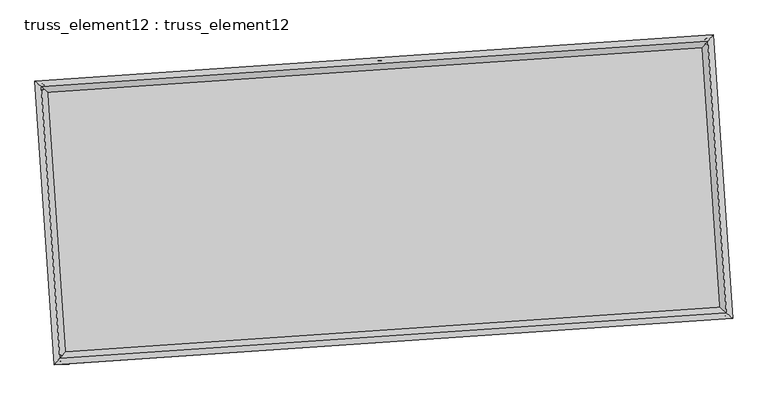
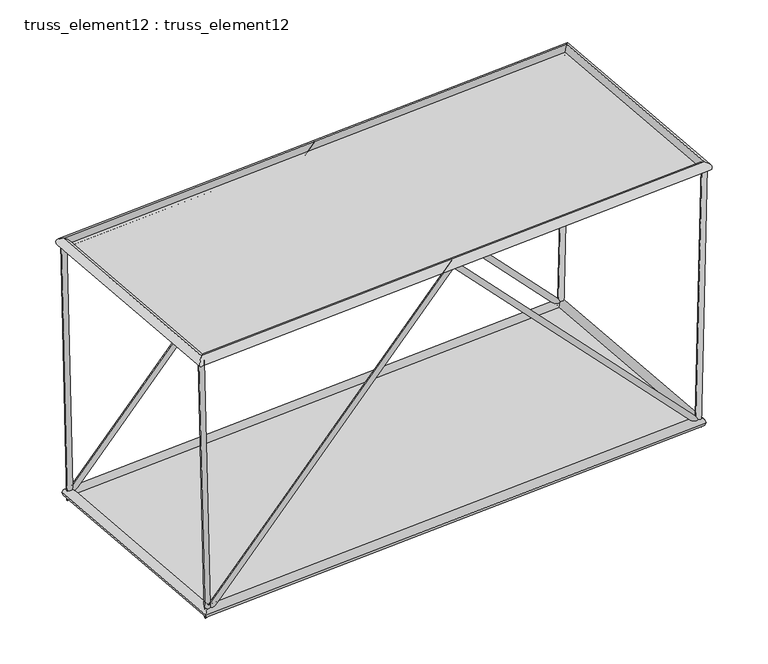
"""IFC4 building model written with IfcOpenShell, lengths in millimetres: plate geometry, truss_element12 : truss_element12."""

import ifcopenshell
import ifcopenshell.guid

model = None  # the IFC model being written
_history = None  # IfcOwnerHistory: only IFC2X3 demands one
_inside = {}  # id of a spatial element -> (the spatial element, [elements in it])
_under = {}  # id of a project, library or spatial element -> (it, [spatial elements below it])
_declared = {}  # id of a project -> (the project, [libraries it declares])
_typed = {}  # id of a type object -> (the type object, [elements of that type])
_made_of = {}  # id of a material, layer set ... -> (it, [elements and type objects made of it])


def new_model(schema):
    """Start an empty IFC model of exactly this schema.

    Asked for "IFC4X3", IfcOpenShell would pick the latest addendum, in which some entities
    have other attributes; the version numbers below select the first issue.
    IFC2X3 requires an IfcOwnerHistory on every rooted entity: one is made here for all.
    """
    global model, _history
    if schema == "IFC4X3":
        model = ifcopenshell.file(schema_version=(4, 3, 0, 0))
    else:
        model = ifcopenshell.file(schema=schema)
    _inside.clear()
    _under.clear()
    _declared.clear()
    _typed.clear()
    _made_of.clear()
    _history = None
    if model.schema == "IFC2X3":
        org = make("IfcOrganization", Name="unknown")
        user = make(
            "IfcPersonAndOrganization",
            ThePerson=make("IfcPerson", FamilyName="unknown"),
            TheOrganization=org,
        )
        app = make(
            "IfcApplication",
            ApplicationDeveloper=org,
            Version="unknown",
            ApplicationFullName="unknown",
            ApplicationIdentifier="unknown",
        )
        _history = make(
            "IfcOwnerHistory",
            OwningUser=user,
            OwningApplication=app,
            ChangeAction="ADDED",
            CreationDate=0,
        )
    return model


def make(cls, **values):
    """One entity of the class cls with the attributes given. An attribute that is None is left unset."""
    return model.create_entity(
        cls, **{name: value for name, value in values.items() if value is not None}
    )


def rooted(cls, **values):
    """An entity with a GlobalId (a new one), such as an element, a storey or a relation."""
    return make(cls, GlobalId=ifcopenshell.guid.new(), OwnerHistory=_history, **values)


def si_unit(unit_type, name, prefix=None):
    """IfcSIUnit, for example si_unit("LENGTHUNIT", "METRE", prefix="MILLI")."""
    return make("IfcSIUnit", UnitType=unit_type, Prefix=prefix, Name=name)


def assignment(units):
    """IfcUnitAssignment: the units of a project."""
    return None if units is None else make("IfcUnitAssignment", Units=units)


def point(xyz):
    """IfcCartesianPoint."""
    return None if xyz is None else make("IfcCartesianPoint", Coordinates=xyz)


def direction(xyz):
    """IfcDirection."""
    return None if xyz is None else make("IfcDirection", DirectionRatios=xyz)


def frame(location, z_axis=None, x_axis=None):
    """IfcAxis2Placement3D, a coordinate frame: its origin and axes. An axis left out is left unset."""
    return make(
        "IfcAxis2Placement3D",
        Location=point(location),
        Axis=direction(z_axis),
        RefDirection=direction(x_axis),
    )


def origin():
    """The frame at (0, 0, 0) with its axes left unset."""
    return frame((0.0, 0.0, 0.0))


def origin_with_axes():
    """The frame at (0, 0, 0) with the z axis (0, 0, 1) and the x axis (1, 0, 0) written out."""
    return frame((0.0, 0.0, 0.0), z_axis=(0.0, 0.0, 1.0), x_axis=(1.0, 0.0, 0.0))


def place(relative_to, where):
    """IfcLocalPlacement: puts the frame where relative to a parent placement (None: the world)."""
    return make(
        "IfcLocalPlacement", PlacementRelTo=relative_to, RelativePlacement=where
    )


def context(
    kind, dimensions, precision=None, world=None, true_north=None, identifier=None
):
    """IfcGeometricRepresentationContext, for example the 3D "Model" context."""
    return make(
        "IfcGeometricRepresentationContext",
        ContextIdentifier=identifier,
        ContextType=kind,
        CoordinateSpaceDimension=dimensions,
        Precision=precision,
        WorldCoordinateSystem=world,
        TrueNorth=true_north,
    )


def project(units=None, contexts=None):
    """IfcProject with its units and contexts."""
    return rooted(
        "IfcProject",
        Name="project",
        RepresentationContexts=contexts,
        UnitsInContext=assignment(units),
    )


def spatial(cls, under=None, at=None, **own):
    """A site, building, storey or space (cls), placed at a placement, below another one or the project."""
    s = rooted(cls, ObjectPlacement=at, **own)
    if under is not None:
        _under.setdefault(under.id(), (under, []))[1].append(s)
    return s


def polyline(points):
    """IfcPolyline through the points."""
    return make("IfcPolyline", Points=[point(p) for p in points])


def circle_curve(where, radius):
    """IfcCircle in the frame where."""
    return make("IfcCircle", Position=where, Radius=radius)


def ellipse_curve(where, semi_axis1, semi_axis2):
    """IfcEllipse in the frame where."""
    return make(
        "IfcEllipse", Position=where, SemiAxis1=semi_axis1, SemiAxis2=semi_axis2
    )


def outline(outer, holes=None, kind="AREA"):
    """IfcArbitraryClosedProfileDef: a profile drawn as a closed curve; with holes, ...WithVoids."""
    if holes is None:
        return make("IfcArbitraryClosedProfileDef", ProfileType=kind, OuterCurve=outer)
    return make(
        "IfcArbitraryProfileDefWithVoids",
        ProfileType=kind,
        OuterCurve=outer,
        InnerCurves=holes,
    )


def extrude(swept, where, along, depth):
    """IfcExtrudedAreaSolid: the profile swept, set in the frame where, extruded along a direction by depth."""
    return make(
        "IfcExtrudedAreaSolid",
        SweptArea=swept,
        Position=where,
        ExtrudedDirection=direction(along),
        Depth=depth,
    )


def shape(context_of_items, identifier, shape_type, items):
    """IfcShapeRepresentation: the items that make up one representation, for example the "Body"."""
    return make(
        "IfcShapeRepresentation",
        ContextOfItems=context_of_items,
        RepresentationIdentifier=identifier,
        RepresentationType=shape_type,
        Items=items,
    )


def source(mapping_origin, context_of_items, identifier, shape_type, items):
    """IfcRepresentationMap: a shape defined once, which mapped items show again and again."""
    return make(
        "IfcRepresentationMap",
        MappingOrigin=mapping_origin,
        MappedRepresentation=shape(context_of_items, identifier, shape_type, items),
    )


def transform(
    local_origin,
    x_axis=None,
    y_axis=None,
    z_axis=None,
    scale=None,
    scale2=None,
    scale3=None,
    uniform=True,
):
    """IfcCartesianTransformationOperator3D, or its non-uniform kind. x_axis, y_axis, z_axis: its Axis1, 2, 3."""
    if uniform:
        return make(
            "IfcCartesianTransformationOperator3D",
            Axis1=direction(x_axis),
            Axis2=direction(y_axis),
            LocalOrigin=point(local_origin),
            Scale=scale,
            Axis3=direction(z_axis),
        )
    return make(
        "IfcCartesianTransformationOperator3DnonUniform",
        Axis1=direction(x_axis),
        Axis2=direction(y_axis),
        LocalOrigin=point(local_origin),
        Scale=scale,
        Axis3=direction(z_axis),
        Scale2=scale2,
        Scale3=scale3,
    )


def mapped(mapping_source, mapping_target):
    """IfcMappedItem: shows the shape of a source again, moved by a transform."""
    return make(
        "IfcMappedItem", MappingSource=mapping_source, MappingTarget=mapping_target
    )


def made_of(thing, what):
    """Note that an element or type object is made of a material, layer set ...; save() writes the relation."""
    if what is not None:
        _made_of.setdefault(what.id(), (what, []))[1].append(thing)
    return thing


def element(
    cls,
    number,
    at=None,
    inside=None,
    cuts=None,
    type_object=None,
    material=None,
    context=None,
    identifier="Body",
    shape_type=None,
    held_by="IfcProductDefinitionShape",
    body=None,
    shapes=None,
    **own,
):
    """One element of the class cls, such as IfcWall. Its Tag is "e" and its number.

    at: its placement. inside: the storey or other place that contains it. cuts: it is an
    opening in that element (IfcRelVoidsElement). A single representation is given by context,
    identifier, shape_type and body (its items); several are given by shapes. held_by: the class
    of the entity that holds the representations. save() writes the other relations.
    """
    e = rooted(cls, Tag="e%d" % number, ObjectPlacement=at, **own)
    if body is not None:
        shapes = [shape(context, identifier, shape_type, body)]
    if shapes is not None:
        e.Representation = make(held_by, Representations=shapes)
    if inside is not None:
        _inside.setdefault(inside.id(), (inside, []))[1].append(e)
    if cuts is not None:
        rooted(
            "IfcRelVoidsElement", RelatingBuildingElement=cuts, RelatedOpeningElement=e
        )
    if type_object is not None:
        _typed.setdefault(type_object.id(), (type_object, []))[1].append(e)
    return made_of(e, material)


def aggregate(whole, parts):
    """IfcRelAggregates: a whole, such as a stair, and the parts it consists of."""
    return rooted("IfcRelAggregates", RelatingObject=whole, RelatedObjects=parts)


def save(model, path):
    """Write the relations noted so far, then the file.

    IfcRelAggregates (storeys below a building ...), IfcRelContainedInSpatialStructure (elements
    in a storey), IfcRelDefinesByType, IfcRelAssociatesMaterial and IfcRelDeclares: one each for
    every whole, place, type object, material and project.
    """
    for whole, parts in _under.values():
        aggregate(whole, parts)
    for where, things in _inside.values():
        rooted(
            "IfcRelContainedInSpatialStructure",
            RelatedElements=things,
            RelatingStructure=where,
        )
    for kind, things in _typed.values():
        rooted("IfcRelDefinesByType", RelatedObjects=things, RelatingType=kind)
    for what, things in _made_of.values():
        rooted("IfcRelAssociatesMaterial", RelatedObjects=things, RelatingMaterial=what)
    for by, libraries in _declared.values():
        rooted("IfcRelDeclares", RelatingContext=by, RelatedDefinitions=libraries)
    model.write(path)


def plane_surface(at):
    """IfcPlane: the flat surface through the origin of the frame at, square to its z axis."""
    return make("IfcPlane", Position=at)


def cylinder_surface(at, radius):
    """IfcCylindricalSurface: all points at the distance radius from the z axis of the frame at."""
    return make("IfcCylindricalSurface", Position=at, Radius=radius)


def advanced_brep(points, edges, surfaces, faces):
    """IfcAdvancedBrep: a solid bounded by faces that lie on surfaces and meet in shared edges.

    An edge is (start, end): straight between two places in points (the first is 0);
    or (start, end, curve); or (start, end, curve, False) where it runs against its curve.
    A face is (place in surfaces, loops), or (place, loops, False) where it looks against
    its surface's normal. A loop lists edges by number (the first is 1), with a minus sign
    where the edge is run from its end to its start. The first loop is the outer one.
    """
    corners = [point(p) for p in points]
    vertices = [make("IfcVertexPoint", VertexGeometry=c) for c in corners]
    made = []
    for start, end, *more in edges:
        made.append(
            make(
                "IfcEdgeCurve",
                EdgeStart=vertices[start],
                EdgeEnd=vertices[end],
                EdgeGeometry=more[0] if more else make("IfcPolyline", Points=[corners[start], corners[end]]),
                SameSense=more[1] if len(more) > 1 else True,
            )
        )
    hull = []
    for where, loops, *sense in faces:
        bounds = []
        for j, loop in enumerate(loops):
            ring = [make("IfcOrientedEdge", EdgeElement=made[abs(k) - 1], Orientation=k > 0) for k in loop]
            bounds.append(
                make(
                    "IfcFaceOuterBound" if j == 0 else "IfcFaceBound",
                    Bound=make("IfcEdgeLoop", EdgeList=ring),
                    Orientation=True,
                )
            )
        hull.append(make("IfcAdvancedFace", Bounds=bounds, FaceSurface=surfaces[where], SameSense=sense[0] if sense else True))
    return make("IfcAdvancedBrep", Outer=make("IfcClosedShell", CfsFaces=hull))


def truss_element12_truss_element12_fedef946(model_context):
    return source(origin(), model_context, "Body", "SolidModel", [
        advanced_brep(
        [(-3782.029021, 2268.2402197, 4999.7937205), (-3881.1049687, 2254.8808593, 4997.4519118), (-3667.7673536, 2276.0312884, 121.2284017), (-3761.2195292, 2263.0553917, -121.2284017), (1063.6545258, 2598.6489605, 5070.7379406), (1064.1036954, 2592.0758396, 4926.5107213), (5795.2031248, 2921.2752732, 121.229281), (5889.5578522, 2921.1052153, -121.229281), (5909.3390115, 2929.0577654, 4999.7954616), (6009.3114208, 2929.2707559, 4997.4562298)],
        [
            (0, 1, circle_curve(frame((-3831.5669949, 2261.5605395, 4998.6228161), z_axis=(-0.02341471068854239, -0.0015965601142035673, 0.9997245632268789), x_axis=(-0.1335941952691201, 0.9910349136664861, -0.0015462485106522157)), 50.0)),
            (1, 0, circle_curve(frame((-3831.5669949, 2261.5605395, 4998.6228161), z_axis=(-0.02341471068854239, -0.0015965601142035673, 0.9997245632268789), x_axis=(-0.1335941952691201, 0.9910349136664861, -0.0015462485106522157)), 50.0)),
            (0, 2),
            (2, 3, ellipse_curve(frame((-3714.4934414, 2269.54334, 0.0), z_axis=(-0.9300661480063914, -0.06341767512013644, 0.36187727037617307), x_axis=(0.3610389440712066, 0.024617873158703073, 0.9322257458282786)), 130.3250571, 50.0)),
            (3, 1),
            (3, 2, ellipse_curve(frame((-3714.4934414, 2269.54334, 0.0), z_axis=(-0.9300661480063914, -0.06341767512013644, 0.36187727037617307), x_axis=(0.3610389440712066, 0.024617873158703073, 0.9322257458282786)), 130.3250571, 50.0)),
            (2, 4),
            (4, 5, ellipse_curve(frame((1063.8791106, 2595.3624001, 4998.6243309), z_axis=(-0.9976833960522568, -0.06802823822716046, -6.7338070324165216e-06), x_axis=(6.718207468311702e-06, 4.5808902877525703e-07, -0.9999999999773279)), 72.2706352, 50.0)),
            (5, 3),
            (5, 4, ellipse_curve(frame((1063.8791106, 2595.3624001, 4998.6243309), z_axis=(-0.9976833960522568, -0.06802823822716046, -6.7338070324165216e-06), x_axis=(6.718207468311702e-06, 4.5808902877525703e-07, -0.9999999999773279)), 72.2706352, 50.0)),
            (4, 6),
            (6, 7, ellipse_curve(frame((5842.3804885, 2921.1902443, 0.0), z_axis=(-0.9300590534640555, -0.06341719137026322, -0.3618955884067292), x_axis=(-0.36105721966614135, -0.02461911930204943, 0.9322186348125355)), 130.3269965, 50.0)),
            (7, 5),
            (7, 6, ellipse_curve(frame((5842.3804885, 2921.1902443, 0.0), z_axis=(-0.9300590534640555, -0.06341719137026322, -0.3618955884067292), x_axis=(-0.36105721966614135, -0.02461911930204943, 0.9322186348125355)), 130.3269965, 50.0)),
            (8, 9, circle_curve(frame((5959.3252161, 2929.1642607, 4998.6258457), z_axis=(0.023388945526827118, 0.0015948032857688488, 0.9997251691488132), x_axis=(-0.002166625472093405, 0.9999964600479803, -0.0015445470442767841)), 50.0)),
            (9, 8, circle_curve(frame((5959.3252161, 2929.1642607, 4998.6258457), z_axis=(0.023388945526827118, 0.0015948032857688488, 0.9997251691488132), x_axis=(-0.002166625472093405, 0.9999964600479803, -0.0015445470442767841)), 50.0)),
            (6, 8),
            (9, 7),
        ],
        [
            plane_surface(frame((-3831.5669949, 2311.5604757, 4998.702666), z_axis=(-0.023414710688541198, -0.0015965601141989434, 0.999724563226879), x_axis=(0.9997258380793066, -3.739324497509243e-05, 0.02341468083005437))),
            cylinder_surface(frame((-3831.5669949, 2261.5605395, 4998.6228161), z_axis=(-0.02341471068854239, -0.0015965601142035673, 0.9997245632268789), x_axis=(-0.1335941952691201, 0.9910349136664861, -0.0015462485106522157)), 50.0),
            cylinder_surface(frame((-3714.4934414, 2269.54334, 0.0), z_axis=(-0.6902363467958819, -0.047064592654016545, -0.7220517361520478), x_axis=(-0.020418619460760453, 0.9987519259602177, -0.04558146959096984)), 50.0),
            cylinder_surface(frame((1063.8791106, 2595.3624001, 4998.6243309), z_axis=(-0.6902460485200185, -0.04706525417770545, 0.722042418665059), x_axis=(-0.11534162865299183, 0.9922794867995385, -0.04558211026839251)), 50.0),
            plane_surface(frame((5959.3252161, 2879.1643243, 4998.7056077), z_axis=(0.023388945526829154, 0.0015948032857737223, 0.9997251691488129), x_axis=(0.999726441196362, -3.731097392289939e-05, -0.023388915766837215))),
            cylinder_surface(frame((5842.3804885, 2921.1902443, 0.0), z_axis=(-0.023388945526827118, -0.0015948032857688488, -0.9997251691488132), x_axis=(-0.002166625472093405, 0.9999964600479803, -0.0015445470442767841)), 50.0),
        ],
        [
            (0, [[1, 2]]),
            (1, [[-1, 3, 4, 5]]),
            (1, [[-2, -5, 6, -3]]),
            (2, [[-4, 7, 8, 9]]),
            (2, [[-6, -9, 10, -7]]),
            (3, [[-8, 11, 12, 13]]),
            (3, [[-10, -13, 14, -11]]),
            (4, [[15, 16]]),
            (5, [[-12, 17, -16, 18]]),
            (5, [[-14, -18, -15, -17]]),
        ],
    ),
        advanced_brep(
        [(-3509.9160681, -1722.4933646, 4999.7937205), (-3608.9920158, -1735.852725, 4997.4519118), (-3395.6544007, -1714.7022959, 121.2284017), (-3489.1065763, -1727.6781926, -121.2284017), (1335.7674788, -1392.0846238, 5070.7379406), (1336.2166483, -1398.6577447, 4926.5107213), (6067.3160777, -1069.4583111, 121.229281), (6161.6708052, -1069.628369, -121.229281), (6181.4519644, -1061.6758189, 4999.7954616), (6281.4243737, -1061.4628284, 4997.4562298)],
        [
            (0, 1, circle_curve(frame((-3559.4540419, -1729.1730448, 4998.6228161), z_axis=(-0.023414710688542402, -0.0015965601142035601, 0.999724563226879), x_axis=(-0.13359419526911945, 0.9910349136664863, -0.001546248510652208)), 50.0)),
            (1, 0, circle_curve(frame((-3559.4540419, -1729.1730448, 4998.6228161), z_axis=(-0.023414710688542402, -0.0015965601142035601, 0.999724563226879), x_axis=(-0.13359419526911945, 0.9910349136664863, -0.001546248510652208)), 50.0)),
            (0, 2),
            (2, 3, ellipse_curve(frame((-3442.3804885, -1721.1902443, 0.0), z_axis=(-0.9300661480063912, -0.06341767512013613, 0.36187727037617334), x_axis=(0.3610389440712068, 0.024617873158702973, 0.9322257458282784)), 130.3250571, 50.0)),
            (3, 1),
            (3, 2, ellipse_curve(frame((-3442.3804885, -1721.1902443, 0.0), z_axis=(-0.9300661480063912, -0.06341767512013613, 0.36187727037617334), x_axis=(0.3610389440712068, 0.024617873158702973, 0.9322257458282784)), 130.3250571, 50.0)),
            (2, 4),
            (4, 5, ellipse_curve(frame((1335.9920636, -1395.3711842, 4998.6243309), z_axis=(-0.997683396052257, -0.0680282382271604, -6.733807032095577e-06), x_axis=(6.718207468465462e-06, 4.5808902903472784e-07, -0.9999999999773279)), 72.2706352, 50.0)),
            (5, 3),
            (5, 4, ellipse_curve(frame((1335.9920636, -1395.3711842, 4998.6243309), z_axis=(-0.997683396052257, -0.0680282382271604, -6.733807032095577e-06), x_axis=(6.718207468465462e-06, 4.5808902903472784e-07, -0.9999999999773279)), 72.2706352, 50.0)),
            (4, 6),
            (6, 7, ellipse_curve(frame((6114.4934414, -1069.54334, 0.0), z_axis=(-0.9300590534640557, -0.06341719137026328, -0.3618955884067287), x_axis=(-0.36105721966614074, -0.02461911930204951, 0.9322186348125356)), 130.3269965, 50.0)),
            (7, 5),
            (7, 6, ellipse_curve(frame((6114.4934414, -1069.54334, 0.0), z_axis=(-0.9300590534640557, -0.06341719137026328, -0.3618955884067287), x_axis=(-0.36105721966614074, -0.02461911930204951, 0.9322186348125356)), 130.3269965, 50.0)),
            (8, 9, circle_curve(frame((6231.4381691, -1061.5693236, 4998.6258457), z_axis=(0.023388945526827663, 0.0015948032857688026, 0.999725169148813), x_axis=(-0.002166625472094084, 0.9999964600479802, -0.001544547044276721)), 50.0)),
            (9, 8, circle_curve(frame((6231.4381691, -1061.5693236, 4998.6258457), z_axis=(0.023388945526827663, 0.0015948032857688026, 0.999725169148813), x_axis=(-0.002166625472094084, 0.9999964600479802, -0.001544547044276721)), 50.0)),
            (6, 8),
            (9, 7),
        ],
        [
            plane_surface(frame((-3559.4540419, -1679.1731086, 4998.702666), z_axis=(-0.023414710688541198, -0.0015965601141989477, 0.999724563226879), x_axis=(0.9997258380793066, -3.739324497509243e-05, 0.02341468083005437))),
            cylinder_surface(frame((-3559.4540419, -1729.1730448, 4998.6228161), z_axis=(-0.023414710688542402, -0.0015965601142035601, 0.999724563226879), x_axis=(-0.13359419526911945, 0.9910349136664863, -0.001546248510652208)), 50.0),
            cylinder_surface(frame((-3442.3804885, -1721.1902443, 0.0), z_axis=(-0.6902363467958823, -0.047064592654016364, -0.7220517361520478), x_axis=(-0.020418619460760457, 0.9987519259602178, -0.04558146959096958)), 50.0),
            cylinder_surface(frame((1335.9920636, -1395.3711842, 4998.6243309), z_axis=(-0.6902460485200181, -0.04706525417770555, 0.7220424186650592), x_axis=(-0.11534162865299175, 0.9922794867995385, -0.04558211026839221)), 50.0),
            plane_surface(frame((6231.4381691, -1111.56926, 4998.7056077), z_axis=(0.02338894552682561, 0.0015948032857737312, 0.9997251691488132), x_axis=(0.9997264411963621, -3.731097392245531e-05, -0.023388915766833666))),
            cylinder_surface(frame((6114.4934414, -1069.54334, 0.0), z_axis=(-0.023388945526827663, -0.0015948032857688026, -0.999725169148813), x_axis=(-0.002166625472094084, 0.9999964600479802, -0.001544547044276721)), 50.0),
        ],
        [
            (0, [[1, 2]]),
            (1, [[-1, 3, 4, 5]]),
            (1, [[-2, -5, 6, -3]]),
            (2, [[-4, 7, 8, 9]]),
            (2, [[-6, -9, 10, -7]]),
            (3, [[-8, 11, 12, 13]]),
            (3, [[-10, -13, 14, -11]]),
            (4, [[15, 16]]),
            (5, [[-12, 17, -16, 18]]),
            (5, [[-14, -18, -15, -17]]),
        ],
    ),
        advanced_brep(
        [(-3559.4532557, -1729.1721734, 4908.6228161), (-3559.4548282, -1729.1739162, 5088.6228161), (-3831.5678921, 2261.5612961, 5088.6228161), (-3831.5660976, 2261.5597829, 4908.6228161), (5959.3259469, 2929.1651283, 5088.6258457), (5959.3244853, 2929.1633931, 4908.6258457), (6231.4390108, -1061.570084, 5088.6258457), (6231.4373273, -1061.5685632, 4908.6258457)],
        [
            (0, 1, ellipse_curve(frame((-3559.4540419, -1729.1730448, 4998.6228161), z_axis=(-0.7535719234054217, 0.657365466278086, -2.182941780963091e-07), x_axis=(-0.65736546627805, -0.7535719234054532, -2.1829417809634472e-07)), 127.2792206, 90.0)),
            (1, 2),
            (2, 3, ellipse_curve(frame((-3831.5669949, 2261.5605395, 4998.6228161), z_axis=(-0.65736546627805, -0.7535719234054532, -2.1829417809637778e-07), x_axis=(0.7535719234054218, -0.6573654662780859, 2.1829417809634224e-07)), 127.2792206, 90.0)),
            (3, 0),
            (1, 0, ellipse_curve(frame((-3559.4540419, -1729.1730448, 4998.6228161), z_axis=(-0.7535719234054217, 0.657365466278086, -2.182941780963091e-07), x_axis=(-0.65736546627805, -0.7535719234054532, -2.1829417809634472e-07)), 127.2792206, 90.0)),
            (3, 2, ellipse_curve(frame((-3831.5669949, 2261.5605395, 4998.6228161), z_axis=(-0.65736546627805, -0.7535719234054532, -2.1829417809637778e-07), x_axis=(0.7535719234054218, -0.6573654662780859, 2.1829417809634224e-07)), 127.2792206, 90.0)),
            (2, 4),
            (4, 5, ellipse_curve(frame((5959.3252161, 2929.1642607, 4998.6258457), z_axis=(-0.7535719234054216, 0.6573654662780861, -2.1829417809637545e-07), x_axis=(-0.6573654662780505, -0.7535719234054526, -2.182941780963446e-07)), 127.2792206, 90.0)),
            (5, 3),
            (5, 4, ellipse_curve(frame((5959.3252161, 2929.1642607, 4998.6258457), z_axis=(-0.7535719234054216, 0.6573654662780861, -2.1829417809637545e-07), x_axis=(-0.6573654662780505, -0.7535719234054526, -2.182941780963446e-07)), 127.2792206, 90.0)),
            (4, 6),
            (6, 7, ellipse_curve(frame((6231.4381691, -1061.5693236, 4998.6258457), z_axis=(0.6573654662780504, 0.7535719234054529, 2.1829417809631145e-07), x_axis=(-0.7535719234054216, 0.6573654662780863, -2.1829417809634234e-07)), 127.2792206, 90.0)),
            (7, 5),
            (7, 6, ellipse_curve(frame((6231.4381691, -1061.5693236, 4998.6258457), z_axis=(0.6573654662780504, 0.7535719234054529, 2.1829417809631145e-07), x_axis=(-0.7535719234054216, 0.6573654662780863, -2.1829417809634234e-07)), 127.2792206, 90.0)),
            (6, 1),
            (0, 7),
        ],
        [
            cylinder_surface(frame((-3559.4540419, -1729.1730448, 4998.6228161), z_axis=(0.06802823822869762, -0.997683396074877, 0.0), x_axis=(-0.9976833960310402, -0.06802823822570855, -9.37427355396142e-06)), 90.0),
            cylinder_surface(frame((-3831.5669949, 2261.5605395, 4998.6228161), z_axis=(-0.9976833960748294, -0.06802823822869407, -3.0871458725096017e-07), x_axis=(-0.06802823822310969, 0.9976833960340703, -9.06555896672317e-06)), 90.0),
            cylinder_surface(frame((5959.3252161, 2929.1642607, 4998.6258457), z_axis=(-0.06802823822869693, 0.9976833960748771, 0.0), x_axis=(0.9976833960366246, 0.06802823822608864, -8.75684437948492e-06)), 90.0),
            cylinder_surface(frame((6231.4381691, -1061.5693236, 4998.6258457), z_axis=(0.9976833960748294, 0.06802823822869393, 3.0871458725091337e-07), x_axis=(0.06802823822869393, -0.9976833960336895, -9.065558966723174e-06)), 90.0),
        ],
        [
            (0, [[1, 2, 3, 4]]),
            (0, [[5, -4, 6, -2]]),
            (1, [[-3, 7, 8, 9]]),
            (1, [[-6, -9, 10, -7]]),
            (2, [[-8, 11, 12, 13]]),
            (2, [[-10, -13, 14, -11]]),
            (3, [[-12, 15, -1, 16]]),
            (3, [[-14, -16, -5, -15]]),
        ],
    ),
        advanced_brep(
        [(-3358.7115243, -1625.2761972, 0.0), (-3526.0494527, -1817.1042913, 0.0), (-3810.4074885, 2353.2123043, 0.0), (-3618.5793943, 2185.8743758, 0.0), (5926.0494527, 3017.1042913, 0.0), (5758.7115243, 2825.2761972, 0.0), (6210.4074885, -1153.2123043, 0.0), (6018.5793943, -985.8743758, 0.0)],
        [
            (0, 1, ellipse_curve(frame((-3442.3804885, -1721.1902443, 0.0), z_axis=(-0.753571923405459, 0.6573654662780796, 0.0), x_axis=(-0.6573654662780796, -0.7535719234054591, 0.0)), 127.2792206, 90.0)),
            (1, 2),
            (2, 3, ellipse_curve(frame((-3714.4934414, 2269.54334, 0.0), z_axis=(-0.6573654662780795, -0.753571923405459, 0.0), x_axis=(0.7535719234054589, -0.6573654662780798, 0.0)), 127.2792206, 90.0)),
            (3, 0),
            (1, 0, ellipse_curve(frame((-3442.3804885, -1721.1902443, 0.0), z_axis=(-0.753571923405459, 0.6573654662780796, 0.0), x_axis=(-0.6573654662780796, -0.7535719234054591, 0.0)), 127.2792206, 90.0)),
            (3, 2, ellipse_curve(frame((-3714.4934414, 2269.54334, 0.0), z_axis=(-0.6573654662780795, -0.753571923405459, 0.0), x_axis=(0.7535719234054589, -0.6573654662780798, 0.0)), 127.2792206, 90.0)),
            (2, 4),
            (4, 5, ellipse_curve(frame((5842.3804885, 2921.1902443, 0.0), z_axis=(-0.753571923405459, 0.6573654662780796, 0.0), x_axis=(-0.6573654662780795, -0.753571923405459, 0.0)), 127.2792206, 90.0)),
            (5, 3),
            (5, 4, ellipse_curve(frame((5842.3804885, 2921.1902443, 0.0), z_axis=(-0.753571923405459, 0.6573654662780796, 0.0), x_axis=(-0.6573654662780795, -0.753571923405459, 0.0)), 127.2792206, 90.0)),
            (4, 6),
            (6, 7, ellipse_curve(frame((6114.4934414, -1069.54334, 0.0), z_axis=(0.6573654662780796, 0.7535719234054591, 0.0), x_axis=(-0.753571923405459, 0.6573654662780795, 0.0)), 127.2792206, 90.0)),
            (7, 5),
            (7, 6, ellipse_curve(frame((6114.4934414, -1069.54334, 0.0), z_axis=(0.6573654662780796, 0.7535719234054591, 0.0), x_axis=(-0.753571923405459, 0.6573654662780795, 0.0)), 127.2792206, 90.0)),
            (6, 1),
            (0, 7),
        ],
        [
            cylinder_surface(frame((-3442.3804885, -1721.1902443, 0.0), z_axis=(0.0680282382287029, -0.9976833960748764, 0.0), x_axis=(-0.9976833960748764, -0.0680282382287029, 0.0)), 90.0),
            cylinder_surface(frame((-3714.4934414, 2269.54334, 0.0), z_axis=(-0.9976833960748764, -0.06802823822870277, 0.0), x_axis=(-0.06802823822870277, 0.9976833960748764, 0.0)), 90.0),
            cylinder_surface(frame((5842.3804885, 2921.1902443, 0.0), z_axis=(-0.06802823822870296, 0.9976833960748764, 0.0), x_axis=(0.9976833960748764, 0.06802823822870296, 0.0)), 90.0),
            cylinder_surface(frame((6114.4934414, -1069.54334, 0.0), z_axis=(0.9976833960748764, 0.06802823822870276, 0.0), x_axis=(0.06802823822870276, -0.9976833960748764, 0.0)), 90.0),
        ],
        [
            (0, [[1, 2, 3, 4]]),
            (0, [[5, -4, 6, -2]]),
            (1, [[-3, 7, 8, 9]]),
            (1, [[-6, -9, 10, -7]]),
            (2, [[-8, 11, 12, 13]]),
            (2, [[-10, -13, 14, -11]]),
            (3, [[-12, 15, -1, 16]]),
            (3, [[-14, -16, -5, -15]]),
        ],
    ),
        extrude(outline(polyline([(-3442.3804885, -1721.1902443), (-3714.4934414, 2269.54334), (5842.3804885, 2921.1902443), (6114.4934414, -1069.54334), (-3442.3804885, -1721.1902443)])), origin_with_axes(), (0.0, 0.0, 1.0), 20.0),
        extrude(outline(polyline([(-2000.0, 4906.8132483), (2000.0000001, 4906.8132484), (2000.0000001, -4906.8132483), (-2000.0, -4906.8132484), (-2000.0, 4906.8132483)])), frame((1199.9355871, 599.9956079, 4998.6243309), z_axis=(-3.0799941782636826e-07, -2.100130948618238e-08, 0.9999999999999524), x_axis=(-0.06802823822870281, 0.9976833960748764, 0.0)), (0.0, 0.0, 1.0), 20.0),
    ])


if __name__ == "__main__":
    model = new_model("IFC4")
    model_context = context("Model", 3, world=origin())
    ifc_project = project(units=[si_unit("LENGTHUNIT", "METRE", prefix="MILLI")], contexts=[model_context])
    site = spatial("IfcSite", under=ifc_project)
    building = spatial("IfcBuilding", under=site)
    placement = place(None, origin())
    truss_element12_truss_element12_shape = truss_element12_truss_element12_fedef946(model_context)
    element("IfcPlate", 1, ObjectType="truss_element12 : truss_element12", at=placement, inside=building, context=model_context, shape_type="MappedRepresentation", body=[
        mapped(truss_element12_truss_element12_shape, transform((0.0, 0.0, 0.0), x_axis=(1.0, 0.0, 0.0), y_axis=(0.0, 1.0, 0.0), z_axis=(0.0, 0.0, 1.0))),
    ])
    save(model, "model.ifc")

# Revit data of these elements
# Type "truss_element12 : truss_element12"
#   steellbar1 = 90 mm
#   steelbar2 = 50 mm
#   offset1 = 5000 mm
#   M = Default Roof
# Element 1 (IfcPlate, "truss_element12 : truss_element12")
#   Materials on its faces: "Default Roof"
# Materials
#   "Default Roof": class "Miscellaneous", colour RGB 0 127 0, transparency 0, Comments = "Rendering appearance not upgraded Rendering appearance not upgraded ", Cost = 0
